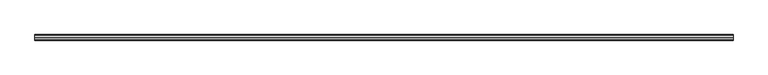
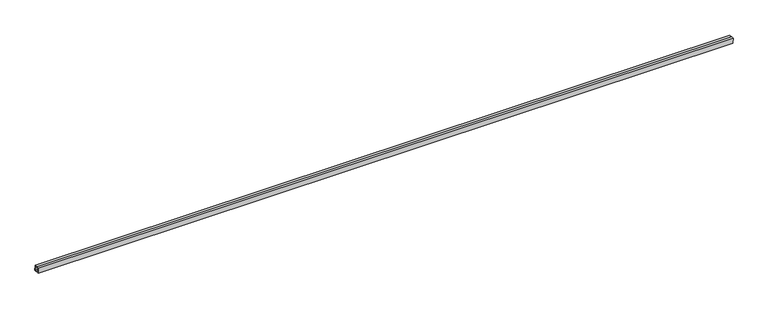
"""IFC4 building model written with IfcOpenShell, lengths in millimetres: proxy geometry, Inner panel:Inner panel:1:Inner panel:1 : Inner panel:Inner panel:300324:2:Inner panel:1:Inner panel:1 : Inner panel:Inner panel:300324:2 : Inner panel:Inner panel:1:Inner panel:1 : Inner panel:Inner panel:300324:300043:15 : Inner panel:Inner panel:1:Inner panel:1 : Inner panel:Inner panel:300324:2:Inner panel:1:Inner panel:1 : Inner panel:Inner panel:300324:2 : Inner panel:Inner panel:1:Inner panel:1 : Inner panel:Inner panel:300324:300043:308120."""

from ifc_helpers import new_model, si_unit, frame, origin, place, context, project, spatial, polyline, outline, extrude, source, transform, mapped, element, save


def generic_models_09dcf16f(model_context):
    return source(origin(), model_context, "Body", "SweptSolid", [
        extrude(outline(polyline([(-577873.8379638, 3996.8505773), (-577855.5975406, 3997.6105949), (-577854.0114169, 3959.5436248), (-577892.078387, 3957.9575011), (-577893.6645107, 3996.0244711), (-577875.4240875, 3996.7844888), (-577875.3249548, 3994.4053031), (-577891.1861923, 3993.7444182), (-577889.7983341, 3960.4358194), (-577856.4897352, 3961.8236777), (-577857.8775935, 3995.1322765), (-577873.7388311, 3994.4713916), (-577873.8379638, 3996.8505773)])), frame((588245.3367239, 0.0, 0.0), z_axis=(1.0, 0.0, 0.0), x_axis=(0.0, 1.0, 0.0)), (0.0, 0.0, 1.0), 4876.8),
    ])


if __name__ == "__main__":
    model = new_model("IFC4")
    model_context = context("Model", 3, world=origin())
    ifc_project = project(units=[si_unit("LENGTHUNIT", "METRE", prefix="MILLI")], contexts=[model_context])
    site = spatial("IfcSite", under=ifc_project)
    building = spatial("IfcBuilding", under=site)
    placement = place(None, origin())
    generic_models_shape = generic_models_09dcf16f(model_context)
    element("IfcBuildingElementProxy", 1, Name="Inner panel:Inner panel:1:Inner panel:1 : Inner panel:Inner panel:300324:2:Inner panel:1:Inner panel:1 : Inner panel:Inner panel:300324:2 : Inner panel:Inner panel:1:Inner panel:1 : Inner panel:Inner panel:300324:300043:15 : Inner panel:Inner panel:1:Inner panel:1 : Inner panel:Inner panel:300324:2:Inner panel:1:Inner panel:1 : Inner panel:Inner panel:300324:2 : Inner panel:Inner panel:1:Inner panel:1 : Inner panel:Inner panel:300324:300043:308120", ObjectType="Inner panel:Inner panel:1:Inner panel:1 : Inner panel:Inner panel:300324:2:Inner panel:1:Inner panel:1 : Inner panel:Inner panel:300324:2 : Inner panel:Inner panel:1:Inner panel:1 : Inner panel:Inner panel:300324:300043:15 : Inner panel:Inner panel:1:Inner panel:1 : Inner panel:Inner panel:300324:2:Inner panel:1:Inner panel:1 : Inner panel:Inner panel:300324:2 : Inner panel:Inner panel:1:Inner panel:1 : Inner panel:Inner panel:300324:300043:308120", at=placement, inside=building, context=model_context, shape_type="MappedRepresentation", body=[
        mapped(generic_models_shape, transform((0.0, 0.0, 0.0), x_axis=(1.0, 0.0, 0.0), y_axis=(0.0, 1.0, 0.0), z_axis=(0.0, 0.0, 1.0))),
    ])
    save(model, "model.ifc")

# Revit data of these elements
# Type "Inner panel:Inner panel:1:Inner panel:1 : Inner panel:Inner panel:300324:2:Inner panel:1:Inner panel:1 : Inner panel:Inner panel:300324:2 : Inner panel:Inner panel:1:Inner panel:1 : Inner panel:Inner panel:300324:300043:15 : Inner panel:Inner panel:1:Inner panel:1 : Inner panel:Inner panel:300324:2:Inner panel:1:Inner panel:1 : Inner panel:Inner panel:300324:2 : Inner panel:Inner panel:1:Inner panel:1 : Inner panel:Inner panel:300324:300043:308120"
#   NameOverride = "Inner panel:Inner panel:1:Inner panel:1 : Inner panel:Inner panel:300324:2:Inner panel:1:Inner panel:1 : Inner panel:Inner panel:300324:2 : Inner panel:Inner panel:1:Inner panel:1 : Inner panel:Inner panel:300324:300043:308120"
#   ObjectTypeOverride = "Inner panel:1:Inner panel:1 : Inner panel:Inner panel:300324:2 : Inner panel:Inner panel:1:Inner panel:1 : Inner panel:Inner panel:300324:300043"
#   Reference = "Inner panel"
#   Tag = "308120"
# Element 1 (IfcBuildingElementProxy, "Inner panel:Inner panel:1:Inner panel:1 : Inner panel:Inner panel:300324:2:Inner panel:1:Inner panel:1 : Inner panel:Inner panel:300324:2 : Inner panel:Inner panel:1:Inner panel:1 : Inner panel:Inner panel:300324:300043:15 : Inner panel:Inner panel:1:Inner panel:1 : Inner panel:Inner panel:300324:2:Inner panel:1:Inner panel:1 : Inner panel:Inner panel:300324:2 : Inner panel:Inner panel:1:Inner panel:1 : Inner panel:Inner panel:300324:300043:308120")
#   Materials on its faces: "1 1/2\" X 1 1/2\" SPLIT-SEAM SQUARE TUBING (~24\" CANTILEVER FROM C.L. OF GLULAM)"
# Materials
#   "1 1/2\" X 1 1/2\" SPLIT-SEAM SQUARE TUBING (~24\" CANTILEVER FROM C.L. OF GLULAM)": class "Unassigned", colour RGB 202 201 200, transparency 0, Cost = 0
